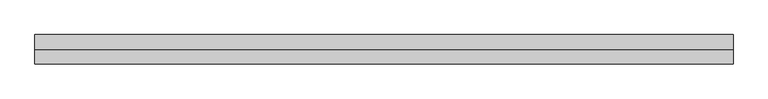
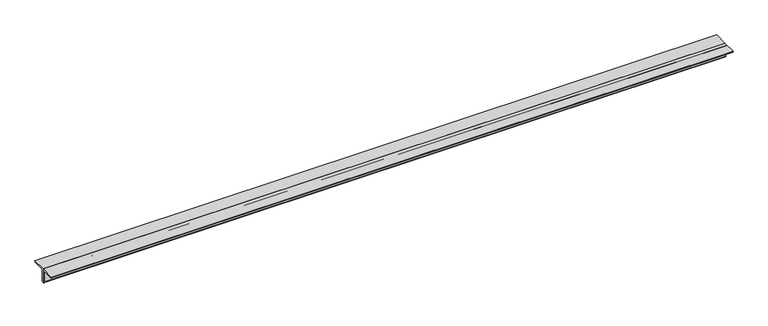
"""IFC4 building model written with IfcOpenShell, lengths in millimetres: member geometry, Steel Framing_2Ls_KS : H_SB_AR_S02_2Ls-100x100x10_VBR1."""

from ifc_helpers import new_model, si_unit, point, frame, frame_2d, origin, place, context, project, spatial, polyline, circle_curve, trimmed, segment, composite_curve, outline, extrude, source, transform, mapped, element, save


def member_028774cf(model_context):
    return source(origin(), model_context, "Body", "SweptSolid", [
        extrude(outline(composite_curve([segment(polyline([(0.0, 28.2), (100.0, 28.2)]), True, "CONTINUOUS"), segment(trimmed(circle_curve(frame_2d((90.0, 28.2)), 10.0), [point((100.0, 28.2))], [point((90.0, 18.2))], False, "CARTESIAN"), True, "CONTINUOUS"), segment(polyline([(90.0, 18.2), (20.0, 18.2)]), True, "CONTINUOUS"), segment(trimmed(circle_curve(frame_2d((20.0, 8.2)), 10.0), [point((20.0, 18.2))], [point((10.0, 8.2))], True, "CARTESIAN"), True, "CONTINUOUS"), segment(polyline([(10.0, 8.2), (10.0, -61.8)]), True, "CONTINUOUS"), segment(trimmed(circle_curve(frame_2d((0.0, -61.8)), 10.0), [point((10.0, -61.8))], [point((0.0, -71.8))], False, "CARTESIAN"), True, "CONTINUOUS"), segment(polyline([(0.0, -71.8), (0.0, 28.2)]), True, "CONTINUOUS")], self_intersect=False)), frame((-2164.6759951, 0.0, 0.0), z_axis=(1.0, 0.0, 0.0), x_axis=(0.0, 1.0, 0.0)), (0.0, 0.0, 1.0), 4755.0114784),
        extrude(outline(composite_curve([segment(polyline([(0.0, 28.2), (0.0, -71.8)]), True, "CONTINUOUS"), segment(trimmed(circle_curve(frame_2d((0.0, -61.8)), 10.0), [point((0.0, -71.8))], [point((-10.0, -61.8))], False, "CARTESIAN"), True, "CONTINUOUS"), segment(polyline([(-10.0, -61.8), (-10.0, 8.2)]), True, "CONTINUOUS"), segment(trimmed(circle_curve(frame_2d((-20.0, 8.2)), 10.0), [point((-10.0, 8.2))], [point((-20.0, 18.2))], True, "CARTESIAN"), True, "CONTINUOUS"), segment(polyline([(-20.0, 18.2), (-90.0, 18.2)]), True, "CONTINUOUS"), segment(trimmed(circle_curve(frame_2d((-90.0, 28.2)), 10.0), [point((-90.0, 18.2))], [point((-100.0, 28.2))], False, "CARTESIAN"), True, "CONTINUOUS"), segment(polyline([(-100.0, 28.2), (0.0, 28.2)]), True, "CONTINUOUS")], self_intersect=False)), frame((-2164.6759951, 0.0, 0.0), z_axis=(1.0, 0.0, 0.0), x_axis=(0.0, 1.0, 0.0)), (0.0, 0.0, 1.0), 4755.0114784),
    ])


if __name__ == "__main__":
    model = new_model("IFC4")
    model_context = context("Model", 3, world=origin())
    ifc_project = project(units=[si_unit("LENGTHUNIT", "METRE", prefix="MILLI")], contexts=[model_context])
    site = spatial("IfcSite", under=ifc_project)
    building = spatial("IfcBuilding", under=site)
    placement = place(None, origin())
    member_shape = member_028774cf(model_context)
    element("IfcMember", 1, ObjectType="Steel Framing_2Ls_KS : H_SB_AR_S02_2Ls-100x100x10_VBR1", at=placement, inside=building, context=model_context, shape_type="MappedRepresentation", body=[
        mapped(member_shape, transform((0.0, 0.0, 0.0), x_axis=(1.0, 0.0, 0.0), y_axis=(0.0, 1.0, 0.0), z_axis=(0.0, 0.0, 1.0))),
    ])
    save(model, "model.ifc")

# Revit data of these elements
# Type "Steel Framing_2Ls_KS : H_SB_AR_S02_2Ls-100x100x10_VBR1"
#   Type Comments = "MAIN"
#   Type Mark = "VBR1"
#   H_SectionID = "2Ls-100x100x10"
#   Assembly Code = "B10"
#   Legs = "LLBB"
#   H_Ratio for Additional Steel Plate = 0.2
#   W = 0
#   Perimeter = 0.80 m²/m
#   Nominal Weight = 29.80 kgf/m
#   Length [instance default] = 1524 mm
#   Space = 0 mm
#   b = 100 mm
#   d = 100 mm
#   t = 10 mm
#   y = 28.2 mm
#   A = 0.0038 m²
#   Structural Material [instance default] = Steel, 45-345
# Element 1 (IfcMember, "Steel Framing_2Ls_KS : H_SB_AR_S02_2Ls-100x100x10_VBR1")
#   Materials on its faces: "Steel, 45-345"
# Materials
#   "Steel, 45-345": class "Metal", colour RGB 189 187 185, transparency 0, Description = "Steel 345 MPa", Cost = 0
